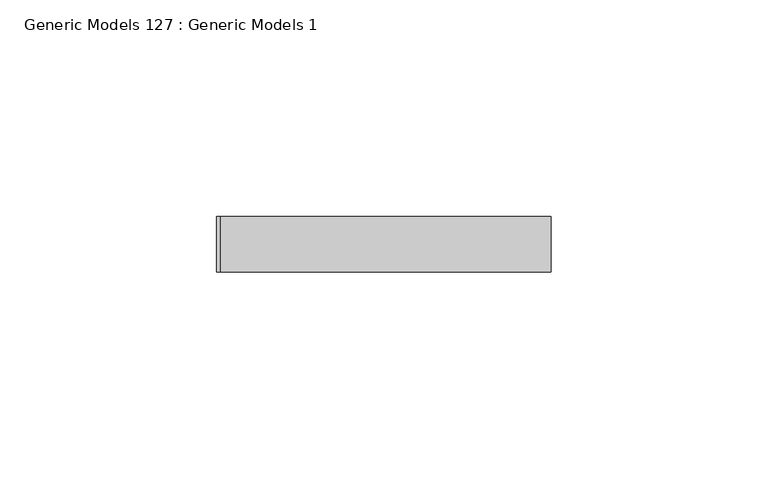
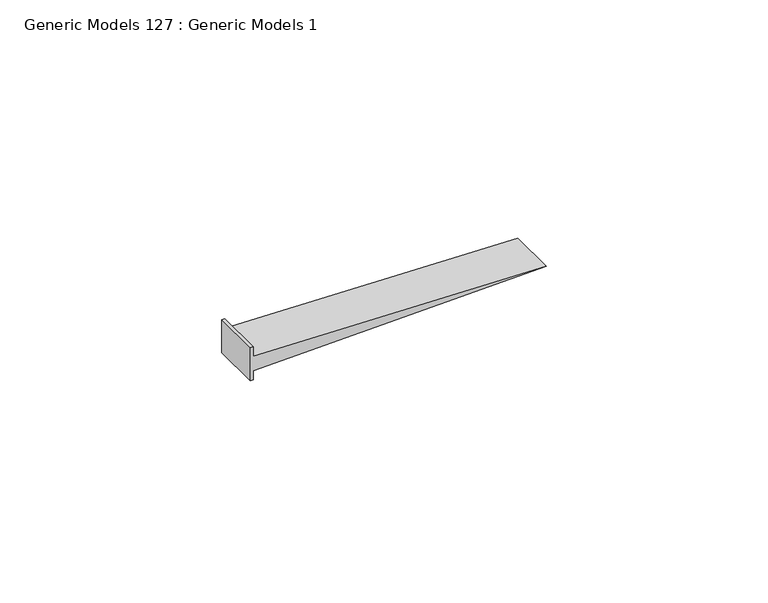
"""IFC4 building model written with IfcOpenShell, lengths in millimetres: proxy geometry, Generic Models 127 : Generic Models 1."""

import ifcopenshell
import ifcopenshell.guid

model = None  # the IFC model being written
_history = None  # IfcOwnerHistory: only IFC2X3 demands one
_inside = {}  # id of a spatial element -> (the spatial element, [elements in it])
_under = {}  # id of a project, library or spatial element -> (it, [spatial elements below it])
_declared = {}  # id of a project -> (the project, [libraries it declares])
_typed = {}  # id of a type object -> (the type object, [elements of that type])
_made_of = {}  # id of a material, layer set ... -> (it, [elements and type objects made of it])


def new_model(schema):
    """Start an empty IFC model of exactly this schema.

    Asked for "IFC4X3", IfcOpenShell would pick the latest addendum, in which some entities
    have other attributes; the version numbers below select the first issue.
    IFC2X3 requires an IfcOwnerHistory on every rooted entity: one is made here for all.
    """
    global model, _history
    if schema == "IFC4X3":
        model = ifcopenshell.file(schema_version=(4, 3, 0, 0))
    else:
        model = ifcopenshell.file(schema=schema)
    _inside.clear()
    _under.clear()
    _declared.clear()
    _typed.clear()
    _made_of.clear()
    _history = None
    if model.schema == "IFC2X3":
        org = make("IfcOrganization", Name="unknown")
        user = make(
            "IfcPersonAndOrganization",
            ThePerson=make("IfcPerson", FamilyName="unknown"),
            TheOrganization=org,
        )
        app = make(
            "IfcApplication",
            ApplicationDeveloper=org,
            Version="unknown",
            ApplicationFullName="unknown",
            ApplicationIdentifier="unknown",
        )
        _history = make(
            "IfcOwnerHistory",
            OwningUser=user,
            OwningApplication=app,
            ChangeAction="ADDED",
            CreationDate=0,
        )
    return model


def make(cls, **values):
    """One entity of the class cls with the attributes given. An attribute that is None is left unset."""
    return model.create_entity(
        cls, **{name: value for name, value in values.items() if value is not None}
    )


def rooted(cls, **values):
    """An entity with a GlobalId (a new one), such as an element, a storey or a relation."""
    return make(cls, GlobalId=ifcopenshell.guid.new(), OwnerHistory=_history, **values)


def si_unit(unit_type, name, prefix=None):
    """IfcSIUnit, for example si_unit("LENGTHUNIT", "METRE", prefix="MILLI")."""
    return make("IfcSIUnit", UnitType=unit_type, Prefix=prefix, Name=name)


def assignment(units):
    """IfcUnitAssignment: the units of a project."""
    return None if units is None else make("IfcUnitAssignment", Units=units)


def point(xyz):
    """IfcCartesianPoint."""
    return None if xyz is None else make("IfcCartesianPoint", Coordinates=xyz)


def direction(xyz):
    """IfcDirection."""
    return None if xyz is None else make("IfcDirection", DirectionRatios=xyz)


def frame(location, z_axis=None, x_axis=None):
    """IfcAxis2Placement3D, a coordinate frame: its origin and axes. An axis left out is left unset."""
    return make(
        "IfcAxis2Placement3D",
        Location=point(location),
        Axis=direction(z_axis),
        RefDirection=direction(x_axis),
    )


def origin():
    """The frame at (0, 0, 0) with its axes left unset."""
    return frame((0.0, 0.0, 0.0))


def place(relative_to, where):
    """IfcLocalPlacement: puts the frame where relative to a parent placement (None: the world)."""
    return make(
        "IfcLocalPlacement", PlacementRelTo=relative_to, RelativePlacement=where
    )


def context(
    kind, dimensions, precision=None, world=None, true_north=None, identifier=None
):
    """IfcGeometricRepresentationContext, for example the 3D "Model" context."""
    return make(
        "IfcGeometricRepresentationContext",
        ContextIdentifier=identifier,
        ContextType=kind,
        CoordinateSpaceDimension=dimensions,
        Precision=precision,
        WorldCoordinateSystem=world,
        TrueNorth=true_north,
    )


def project(units=None, contexts=None):
    """IfcProject with its units and contexts."""
    return rooted(
        "IfcProject",
        Name="project",
        RepresentationContexts=contexts,
        UnitsInContext=assignment(units),
    )


def spatial(cls, under=None, at=None, **own):
    """A site, building, storey or space (cls), placed at a placement, below another one or the project."""
    s = rooted(cls, ObjectPlacement=at, **own)
    if under is not None:
        _under.setdefault(under.id(), (under, []))[1].append(s)
    return s


def polyline(points):
    """IfcPolyline through the points."""
    return make("IfcPolyline", Points=[point(p) for p in points])


def outline(outer, holes=None, kind="AREA"):
    """IfcArbitraryClosedProfileDef: a profile drawn as a closed curve; with holes, ...WithVoids."""
    if holes is None:
        return make("IfcArbitraryClosedProfileDef", ProfileType=kind, OuterCurve=outer)
    return make(
        "IfcArbitraryProfileDefWithVoids",
        ProfileType=kind,
        OuterCurve=outer,
        InnerCurves=holes,
    )


def extrude(swept, where, along, depth):
    """IfcExtrudedAreaSolid: the profile swept, set in the frame where, extruded along a direction by depth."""
    return make(
        "IfcExtrudedAreaSolid",
        SweptArea=swept,
        Position=where,
        ExtrudedDirection=direction(along),
        Depth=depth,
    )


def shape(context_of_items, identifier, shape_type, items):
    """IfcShapeRepresentation: the items that make up one representation, for example the "Body"."""
    return make(
        "IfcShapeRepresentation",
        ContextOfItems=context_of_items,
        RepresentationIdentifier=identifier,
        RepresentationType=shape_type,
        Items=items,
    )


def source(mapping_origin, context_of_items, identifier, shape_type, items):
    """IfcRepresentationMap: a shape defined once, which mapped items show again and again."""
    return make(
        "IfcRepresentationMap",
        MappingOrigin=mapping_origin,
        MappedRepresentation=shape(context_of_items, identifier, shape_type, items),
    )


def transform(
    local_origin,
    x_axis=None,
    y_axis=None,
    z_axis=None,
    scale=None,
    scale2=None,
    scale3=None,
    uniform=True,
):
    """IfcCartesianTransformationOperator3D, or its non-uniform kind. x_axis, y_axis, z_axis: its Axis1, 2, 3."""
    if uniform:
        return make(
            "IfcCartesianTransformationOperator3D",
            Axis1=direction(x_axis),
            Axis2=direction(y_axis),
            LocalOrigin=point(local_origin),
            Scale=scale,
            Axis3=direction(z_axis),
        )
    return make(
        "IfcCartesianTransformationOperator3DnonUniform",
        Axis1=direction(x_axis),
        Axis2=direction(y_axis),
        LocalOrigin=point(local_origin),
        Scale=scale,
        Axis3=direction(z_axis),
        Scale2=scale2,
        Scale3=scale3,
    )


def mapped(mapping_source, mapping_target):
    """IfcMappedItem: shows the shape of a source again, moved by a transform."""
    return make(
        "IfcMappedItem", MappingSource=mapping_source, MappingTarget=mapping_target
    )


def made_of(thing, what):
    """Note that an element or type object is made of a material, layer set ...; save() writes the relation."""
    if what is not None:
        _made_of.setdefault(what.id(), (what, []))[1].append(thing)
    return thing


def element(
    cls,
    number,
    at=None,
    inside=None,
    cuts=None,
    type_object=None,
    material=None,
    context=None,
    identifier="Body",
    shape_type=None,
    held_by="IfcProductDefinitionShape",
    body=None,
    shapes=None,
    **own,
):
    """One element of the class cls, such as IfcWall. Its Tag is "e" and its number.

    at: its placement. inside: the storey or other place that contains it. cuts: it is an
    opening in that element (IfcRelVoidsElement). A single representation is given by context,
    identifier, shape_type and body (its items); several are given by shapes. held_by: the class
    of the entity that holds the representations. save() writes the other relations.
    """
    e = rooted(cls, Tag="e%d" % number, ObjectPlacement=at, **own)
    if body is not None:
        shapes = [shape(context, identifier, shape_type, body)]
    if shapes is not None:
        e.Representation = make(held_by, Representations=shapes)
    if inside is not None:
        _inside.setdefault(inside.id(), (inside, []))[1].append(e)
    if cuts is not None:
        rooted(
            "IfcRelVoidsElement", RelatingBuildingElement=cuts, RelatedOpeningElement=e
        )
    if type_object is not None:
        _typed.setdefault(type_object.id(), (type_object, []))[1].append(e)
    return made_of(e, material)


def aggregate(whole, parts):
    """IfcRelAggregates: a whole, such as a stair, and the parts it consists of."""
    return rooted("IfcRelAggregates", RelatingObject=whole, RelatedObjects=parts)


def save(model, path):
    """Write the relations noted so far, then the file.

    IfcRelAggregates (storeys below a building ...), IfcRelContainedInSpatialStructure (elements
    in a storey), IfcRelDefinesByType, IfcRelAssociatesMaterial and IfcRelDeclares: one each for
    every whole, place, type object, material and project.
    """
    for whole, parts in _under.values():
        aggregate(whole, parts)
    for where, things in _inside.values():
        rooted(
            "IfcRelContainedInSpatialStructure",
            RelatedElements=things,
            RelatingStructure=where,
        )
    for kind, things in _typed.values():
        rooted("IfcRelDefinesByType", RelatedObjects=things, RelatingType=kind)
    for what, things in _made_of.values():
        rooted("IfcRelAssociatesMaterial", RelatedObjects=things, RelatingMaterial=what)
    for by, libraries in _declared.values():
        rooted("IfcRelDeclares", RelatingContext=by, RelatedDefinitions=libraries)
    model.write(path)


def generic_models_127_generic_models_1_a25d7756(model_context):
    return source(origin(), model_context, "Body", "SweptSolid", [
        extrude(outline(polyline([(2414.3721662, 49675.25625), (2405.2789662, 49675.25625), (2405.2789662, 49676.05), (2407.8288298, 49676.05), (2409.8255662, 49752.25), (2411.8223026, 49676.05), (2414.3721662, 49676.05), (2414.3721662, 49675.25625)])), frame((0.0, 565.15, 0.0), z_axis=(0.0, 1.0, 0.0), x_axis=(0.0, 0.0, 1.0)), (0.0, 0.0, 1.0), 12.7),
    ])


if __name__ == "__main__":
    model = new_model("IFC4")
    model_context = context("Model", 3, world=origin())
    ifc_project = project(units=[si_unit("LENGTHUNIT", "METRE", prefix="MILLI")], contexts=[model_context])
    site = spatial("IfcSite", under=ifc_project)
    building = spatial("IfcBuilding", under=site)
    placement = place(None, origin())
    generic_models_127_generic_models_1_shape = generic_models_127_generic_models_1_a25d7756(model_context)
    element("IfcBuildingElementProxy", 1, Name="Generic Models 127 : Generic Models 1", ObjectType="Generic Models 127 : Generic Models 1", at=placement, inside=building, context=model_context, shape_type="MappedRepresentation", body=[
        mapped(generic_models_127_generic_models_1_shape, transform((0.0, 0.0, 0.0), x_axis=(1.0, 0.0, 0.0), y_axis=(0.0, 1.0, 0.0), z_axis=(0.0, 0.0, 1.0))),
    ])
    save(model, "model.ifc")

# Revit data of these elements
# Element 1 (IfcBuildingElementProxy, "Generic Models 127 : Generic Models 1")
#   Materials on its faces: "ATTACH GYPSUM BOARD TO STUDS AND NOT TO TOP TRACK"
# Materials
#   "ATTACH GYPSUM BOARD TO STUDS AND NOT TO TOP TRACK": class "Generic", colour RGB 48 48 48, transparency 0, Cost = 0
